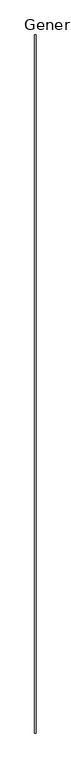
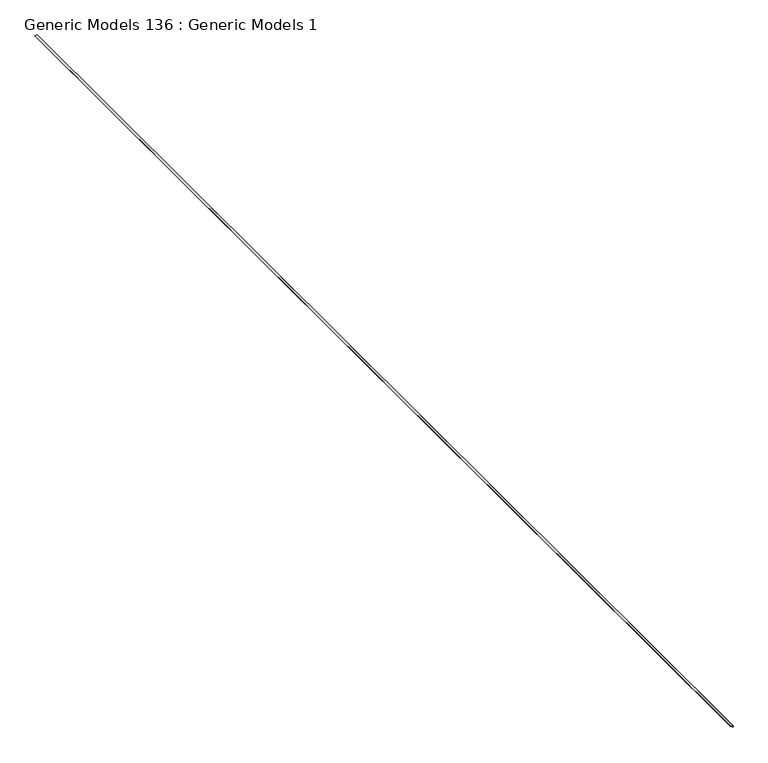
"""IFC4 building model written with IfcOpenShell, lengths in millimetres: proxy geometry, Generic Models 136 : Generic Models 1."""

from ifc_helpers import new_model, si_unit, frame, origin, place, context, project, spatial, polyline, outline, extrude, source, transform, mapped, element, save


def generic_models_136_generic_models_1_a9636d30(model_context):
    return source(origin(), model_context, "Body", "SweptSolid", [
        extrude(outline(polyline([(126312.2670671, 7259.9960984), (126334.4920671, 7259.9960984), (126334.4920671, 7221.8960984), (126333.2220671, 7221.8960984), (126333.2220671, 7258.7260984), (126313.5370671, 7258.7260984), (126313.5370671, 7256.5162984), (126315.2695234, 7256.5162984), (126315.2695234, 7255.2462984), (126312.2670671, 7255.2462984), (126312.2670671, 7259.9960984)])), frame((0.0, -7068.1230338, 0.0), z_axis=(0.0, 1.0, 0.0), x_axis=(0.0, 0.0, 1.0)), (0.0, 0.0, 1.0), 19050.0),
    ])


if __name__ == "__main__":
    model = new_model("IFC4")
    model_context = context("Model", 3, world=origin())
    ifc_project = project(units=[si_unit("LENGTHUNIT", "METRE", prefix="MILLI")], contexts=[model_context])
    site = spatial("IfcSite", under=ifc_project)
    building = spatial("IfcBuilding", under=site)
    placement = place(None, origin())
    generic_models_136_generic_models_1_shape = generic_models_136_generic_models_1_a9636d30(model_context)
    element("IfcBuildingElementProxy", 1, Name="Generic Models 136 : Generic Models 1", ObjectType="Generic Models 136 : Generic Models 1", at=placement, inside=building, context=model_context, shape_type="MappedRepresentation", body=[
        mapped(generic_models_136_generic_models_1_shape, transform((0.0, 0.0, 0.0), x_axis=(1.0, 0.0, 0.0), y_axis=(0.0, 1.0, 0.0), z_axis=(0.0, 0.0, 1.0))),
    ])
    save(model, "model.ifc")

# Revit data of these elements
# Element 1 (IfcBuildingElementProxy, "Generic Models 136 : Generic Models 1")
#   Materials on its faces: "_CONTINUOUS 16 GA. COPPER  J BEAD"
# Materials
#   "_CONTINUOUS 16 GA. COPPER  J BEAD": class "Generic", colour RGB 253 192 103, transparency 0, Cost = 0
